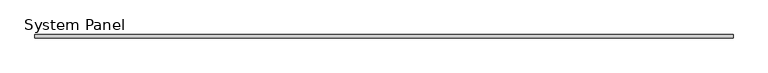
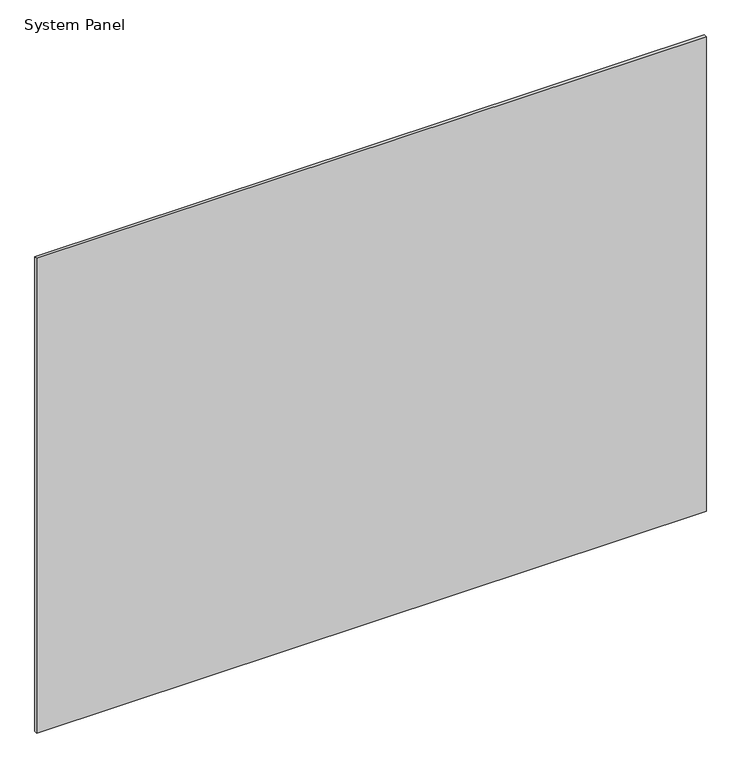
"""IFC4 building model written with IfcOpenShell, lengths in millimetres: plate geometry, System Panel : WWm-Glass-20mm-10mmOffset."""

import ifcopenshell
import ifcopenshell.guid

model = None  # the IFC model being written
_history = None  # IfcOwnerHistory: only IFC2X3 demands one
_inside = {}  # id of a spatial element -> (the spatial element, [elements in it])
_under = {}  # id of a project, library or spatial element -> (it, [spatial elements below it])
_declared = {}  # id of a project -> (the project, [libraries it declares])
_typed = {}  # id of a type object -> (the type object, [elements of that type])
_made_of = {}  # id of a material, layer set ... -> (it, [elements and type objects made of it])


def new_model(schema):
    """Start an empty IFC model of exactly this schema.

    Asked for "IFC4X3", IfcOpenShell would pick the latest addendum, in which some entities
    have other attributes; the version numbers below select the first issue.
    IFC2X3 requires an IfcOwnerHistory on every rooted entity: one is made here for all.
    """
    global model, _history
    if schema == "IFC4X3":
        model = ifcopenshell.file(schema_version=(4, 3, 0, 0))
    else:
        model = ifcopenshell.file(schema=schema)
    _inside.clear()
    _under.clear()
    _declared.clear()
    _typed.clear()
    _made_of.clear()
    _history = None
    if model.schema == "IFC2X3":
        org = make("IfcOrganization", Name="unknown")
        user = make(
            "IfcPersonAndOrganization",
            ThePerson=make("IfcPerson", FamilyName="unknown"),
            TheOrganization=org,
        )
        app = make(
            "IfcApplication",
            ApplicationDeveloper=org,
            Version="unknown",
            ApplicationFullName="unknown",
            ApplicationIdentifier="unknown",
        )
        _history = make(
            "IfcOwnerHistory",
            OwningUser=user,
            OwningApplication=app,
            ChangeAction="ADDED",
            CreationDate=0,
        )
    return model


def make(cls, **values):
    """One entity of the class cls with the attributes given. An attribute that is None is left unset."""
    return model.create_entity(
        cls, **{name: value for name, value in values.items() if value is not None}
    )


def rooted(cls, **values):
    """An entity with a GlobalId (a new one), such as an element, a storey or a relation."""
    return make(cls, GlobalId=ifcopenshell.guid.new(), OwnerHistory=_history, **values)


def si_unit(unit_type, name, prefix=None):
    """IfcSIUnit, for example si_unit("LENGTHUNIT", "METRE", prefix="MILLI")."""
    return make("IfcSIUnit", UnitType=unit_type, Prefix=prefix, Name=name)


def assignment(units):
    """IfcUnitAssignment: the units of a project."""
    return None if units is None else make("IfcUnitAssignment", Units=units)


def point(xyz):
    """IfcCartesianPoint."""
    return None if xyz is None else make("IfcCartesianPoint", Coordinates=xyz)


def direction(xyz):
    """IfcDirection."""
    return None if xyz is None else make("IfcDirection", DirectionRatios=xyz)


def frame(location, z_axis=None, x_axis=None):
    """IfcAxis2Placement3D, a coordinate frame: its origin and axes. An axis left out is left unset."""
    return make(
        "IfcAxis2Placement3D",
        Location=point(location),
        Axis=direction(z_axis),
        RefDirection=direction(x_axis),
    )


def origin():
    """The frame at (0, 0, 0) with its axes left unset."""
    return frame((0.0, 0.0, 0.0))


def origin_with_axes():
    """The frame at (0, 0, 0) with the z axis (0, 0, 1) and the x axis (1, 0, 0) written out."""
    return frame((0.0, 0.0, 0.0), z_axis=(0.0, 0.0, 1.0), x_axis=(1.0, 0.0, 0.0))


def place(relative_to, where):
    """IfcLocalPlacement: puts the frame where relative to a parent placement (None: the world)."""
    return make(
        "IfcLocalPlacement", PlacementRelTo=relative_to, RelativePlacement=where
    )


def context(
    kind, dimensions, precision=None, world=None, true_north=None, identifier=None
):
    """IfcGeometricRepresentationContext, for example the 3D "Model" context."""
    return make(
        "IfcGeometricRepresentationContext",
        ContextIdentifier=identifier,
        ContextType=kind,
        CoordinateSpaceDimension=dimensions,
        Precision=precision,
        WorldCoordinateSystem=world,
        TrueNorth=true_north,
    )


def project(units=None, contexts=None):
    """IfcProject with its units and contexts."""
    return rooted(
        "IfcProject",
        Name="project",
        RepresentationContexts=contexts,
        UnitsInContext=assignment(units),
    )


def spatial(cls, under=None, at=None, **own):
    """A site, building, storey or space (cls), placed at a placement, below another one or the project."""
    s = rooted(cls, ObjectPlacement=at, **own)
    if under is not None:
        _under.setdefault(under.id(), (under, []))[1].append(s)
    return s


def polyline(points):
    """IfcPolyline through the points."""
    return make("IfcPolyline", Points=[point(p) for p in points])


def outline(outer, holes=None, kind="AREA"):
    """IfcArbitraryClosedProfileDef: a profile drawn as a closed curve; with holes, ...WithVoids."""
    if holes is None:
        return make("IfcArbitraryClosedProfileDef", ProfileType=kind, OuterCurve=outer)
    return make(
        "IfcArbitraryProfileDefWithVoids",
        ProfileType=kind,
        OuterCurve=outer,
        InnerCurves=holes,
    )


def extrude(swept, where, along, depth):
    """IfcExtrudedAreaSolid: the profile swept, set in the frame where, extruded along a direction by depth."""
    return make(
        "IfcExtrudedAreaSolid",
        SweptArea=swept,
        Position=where,
        ExtrudedDirection=direction(along),
        Depth=depth,
    )


def shape(context_of_items, identifier, shape_type, items):
    """IfcShapeRepresentation: the items that make up one representation, for example the "Body"."""
    return make(
        "IfcShapeRepresentation",
        ContextOfItems=context_of_items,
        RepresentationIdentifier=identifier,
        RepresentationType=shape_type,
        Items=items,
    )


def source(mapping_origin, context_of_items, identifier, shape_type, items):
    """IfcRepresentationMap: a shape defined once, which mapped items show again and again."""
    return make(
        "IfcRepresentationMap",
        MappingOrigin=mapping_origin,
        MappedRepresentation=shape(context_of_items, identifier, shape_type, items),
    )


def transform(
    local_origin,
    x_axis=None,
    y_axis=None,
    z_axis=None,
    scale=None,
    scale2=None,
    scale3=None,
    uniform=True,
):
    """IfcCartesianTransformationOperator3D, or its non-uniform kind. x_axis, y_axis, z_axis: its Axis1, 2, 3."""
    if uniform:
        return make(
            "IfcCartesianTransformationOperator3D",
            Axis1=direction(x_axis),
            Axis2=direction(y_axis),
            LocalOrigin=point(local_origin),
            Scale=scale,
            Axis3=direction(z_axis),
        )
    return make(
        "IfcCartesianTransformationOperator3DnonUniform",
        Axis1=direction(x_axis),
        Axis2=direction(y_axis),
        LocalOrigin=point(local_origin),
        Scale=scale,
        Axis3=direction(z_axis),
        Scale2=scale2,
        Scale3=scale3,
    )


def mapped(mapping_source, mapping_target):
    """IfcMappedItem: shows the shape of a source again, moved by a transform."""
    return make(
        "IfcMappedItem", MappingSource=mapping_source, MappingTarget=mapping_target
    )


def made_of(thing, what):
    """Note that an element or type object is made of a material, layer set ...; save() writes the relation."""
    if what is not None:
        _made_of.setdefault(what.id(), (what, []))[1].append(thing)
    return thing


def element(
    cls,
    number,
    at=None,
    inside=None,
    cuts=None,
    type_object=None,
    material=None,
    context=None,
    identifier="Body",
    shape_type=None,
    held_by="IfcProductDefinitionShape",
    body=None,
    shapes=None,
    **own,
):
    """One element of the class cls, such as IfcWall. Its Tag is "e" and its number.

    at: its placement. inside: the storey or other place that contains it. cuts: it is an
    opening in that element (IfcRelVoidsElement). A single representation is given by context,
    identifier, shape_type and body (its items); several are given by shapes. held_by: the class
    of the entity that holds the representations. save() writes the other relations.
    """
    e = rooted(cls, Tag="e%d" % number, ObjectPlacement=at, **own)
    if body is not None:
        shapes = [shape(context, identifier, shape_type, body)]
    if shapes is not None:
        e.Representation = make(held_by, Representations=shapes)
    if inside is not None:
        _inside.setdefault(inside.id(), (inside, []))[1].append(e)
    if cuts is not None:
        rooted(
            "IfcRelVoidsElement", RelatingBuildingElement=cuts, RelatedOpeningElement=e
        )
    if type_object is not None:
        _typed.setdefault(type_object.id(), (type_object, []))[1].append(e)
    return made_of(e, material)


def aggregate(whole, parts):
    """IfcRelAggregates: a whole, such as a stair, and the parts it consists of."""
    return rooted("IfcRelAggregates", RelatingObject=whole, RelatedObjects=parts)


def save(model, path):
    """Write the relations noted so far, then the file.

    IfcRelAggregates (storeys below a building ...), IfcRelContainedInSpatialStructure (elements
    in a storey), IfcRelDefinesByType, IfcRelAssociatesMaterial and IfcRelDeclares: one each for
    every whole, place, type object, material and project.
    """
    for whole, parts in _under.values():
        aggregate(whole, parts)
    for where, things in _inside.values():
        rooted(
            "IfcRelContainedInSpatialStructure",
            RelatedElements=things,
            RelatingStructure=where,
        )
    for kind, things in _typed.values():
        rooted("IfcRelDefinesByType", RelatedObjects=things, RelatingType=kind)
    for what, things in _made_of.values():
        rooted("IfcRelAssociatesMaterial", RelatedObjects=things, RelatingMaterial=what)
    for by, libraries in _declared.values():
        rooted("IfcRelDeclares", RelatingContext=by, RelatedDefinitions=libraries)
    model.write(path)


def system_panel_75acd469(model_context):
    return source(origin(), model_context, "Body", "SweptSolid", [
        extrude(outline(polyline([(2236.114364, 0.0), (-2236.114364, 0.0), (-2236.114364, 20.0), (2236.114364, 20.0), (2236.114364, 0.0)])), origin_with_axes(), (0.0, 0.0, 1.0), 3350.0),
    ])


if __name__ == "__main__":
    model = new_model("IFC4")
    model_context = context("Model", 3, world=origin())
    ifc_project = project(units=[si_unit("LENGTHUNIT", "METRE", prefix="MILLI")], contexts=[model_context])
    site = spatial("IfcSite", under=ifc_project)
    building = spatial("IfcBuilding", under=site)
    placement = place(None, origin())
    system_panel_shape = system_panel_75acd469(model_context)
    element("IfcPlate", 1, ObjectType="System Panel : WWm-Glass-20mm-10mmOffset", at=placement, inside=building, context=model_context, shape_type="MappedRepresentation", body=[
        mapped(system_panel_shape, transform((0.0, 0.0, 0.0), x_axis=(1.0, 0.0, 0.0), y_axis=(0.0, 1.0, 0.0), z_axis=(0.0, 0.0, 1.0))),
    ])
    save(model, "model.ifc")

# Revit data of these elements
# Type "System Panel : WWm-Glass-20mm-10mmOffset"
#   Finish = ""
# Element 1 (IfcPlate, "System Panel : WWm-Glass-20mm-10mmOffset")
#   Materials on its faces: "WW-EC-GL-Storefront"
# Materials
#   "WW-EC-GL-Storefront": class "Glass", colour RGB 236 240 239, transparency 0.85, Description = "Storefront Glass", Cost = 0
